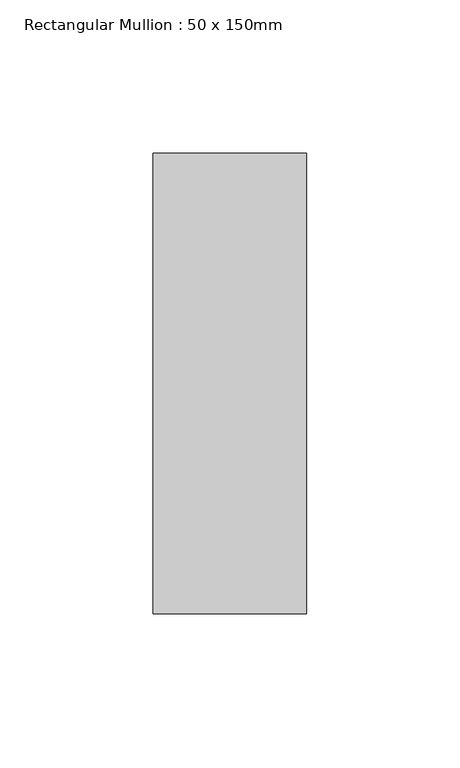
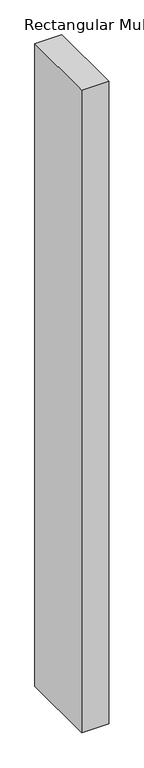
"""IFC4 building model written with IfcOpenShell, lengths in millimetres: member geometry, Rectangular Mullion : 50 x 150mm."""

from ifc_helpers import new_model, si_unit, frame, origin, place, context, project, spatial, polyline, outline, extrude, source, transform, mapped, element, save


def rectangular_mullion_50_x_150mm_5b019a6c(model_context):
    return source(origin(), model_context, "Body", "SweptSolid", [
        extrude(outline(polyline([(0.0, 75.0), (0.0, -75.0), (-50.0, -75.0), (-50.0, 75.0), (0.0, 75.0)])), frame((0.0, 0.0, -1258.3333333), z_axis=(0.0, 0.0, 1.0), x_axis=(1.0, 0.0, 0.0)), (0.0, 0.0, 1.0), 1258.3333333),
    ])


if __name__ == "__main__":
    model = new_model("IFC4")
    model_context = context("Model", 3, world=origin())
    ifc_project = project(units=[si_unit("LENGTHUNIT", "METRE", prefix="MILLI")], contexts=[model_context])
    site = spatial("IfcSite", under=ifc_project)
    building = spatial("IfcBuilding", under=site)
    placement = place(None, origin())
    rectangular_mullion_50_x_150mm_shape = rectangular_mullion_50_x_150mm_5b019a6c(model_context)
    element("IfcMember", 1, ObjectType="Rectangular Mullion : 50 x 150mm", at=placement, inside=building, context=model_context, shape_type="MappedRepresentation", body=[
        mapped(rectangular_mullion_50_x_150mm_shape, transform((0.0, 0.0, 0.0), x_axis=(1.0, 0.0, 0.0), y_axis=(0.0, 1.0, 0.0), z_axis=(0.0, 0.0, 1.0))),
    ])
    save(model, "model.ifc")

# Revit data of these elements
# Type "Rectangular Mullion : 50 x 150mm"
#   built-in parameter 1007304 = 0.492126 (stored number, unit not read)
#   built-in parameter 1007301 = 0.082021 (stored number, unit not read)
#   built-in parameter 1007300 = 0.082021 (stored number, unit not read)
# Element 1 (IfcMember, "Rectangular Mullion : 50 x 150mm")
#   Materials on its faces: "Metal - Aluminium"
# Materials
#   "Metal - Aluminium": class "Metal", colour RGB 247 247 247, transparency 0
